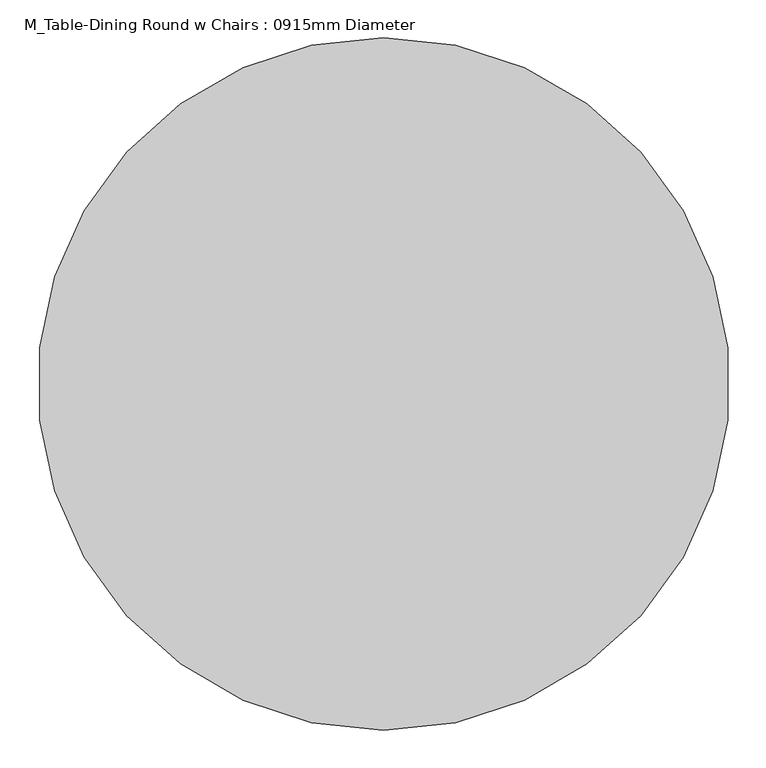
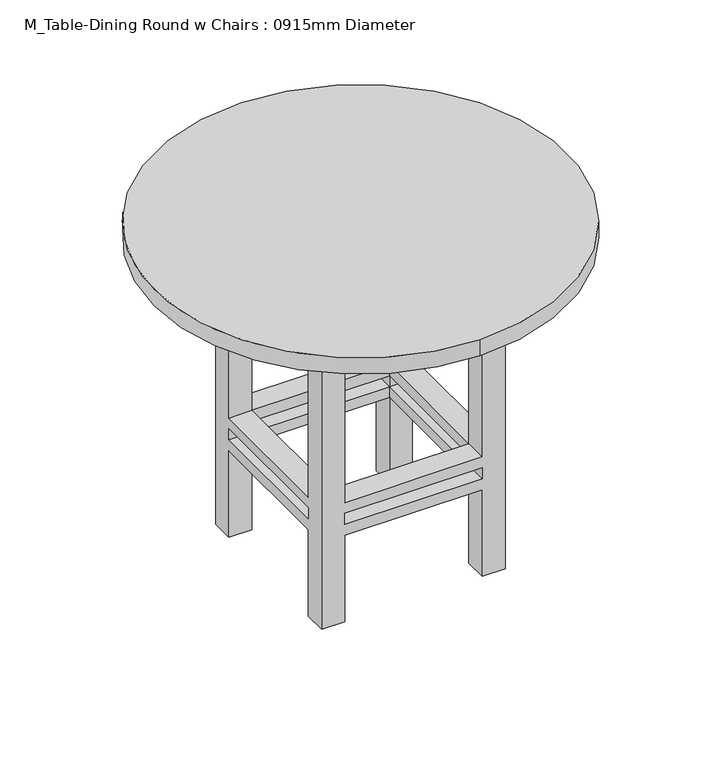
"""IFC4 building model written with IfcOpenShell, lengths in millimetres: furniture geometry, M_Table-Dining Round w Chairs : 0915mm Diameter."""

from ifc_helpers import new_model, si_unit, point, frame, frame_2d, origin, place, context, project, spatial, polyline, circle_curve, trimmed, segment, composite_curve, outline, extrude, faceted_brep, source, transform, mapped, element, save


def m_table_dining_round_w_chairs_0915mm_diameter_5defa876(model_context):
    return source(origin(), model_context, "Body", "SolidModel", [
        faceted_brep([(-48.8680328, 18.4713115, 647.7), (-99.6680328, 18.4713115, 647.7), (-99.6680328, -32.3286885, 647.7), (-48.8680328, -32.3286885, 647.7), (256.2319672, 18.4713115, 647.7), (256.2319672, -32.3286885, 647.7), (307.0319672, -32.3286885, 647.7), (307.0319672, 18.4713115, 647.7), (256.2319672, -388.2286885, 647.7), (307.0319672, -388.2286885, 647.7), (307.0319672, -337.4286885, 647.7), (256.2319672, -337.4286885, 647.7), (-48.8680328, -388.2286885, 647.7), (-48.8680328, -337.4286885, 647.7), (-99.6680328, -337.4286885, 647.7), (-99.6680328, -388.2286885, 647.7), (-48.8680328, 18.4713115, 0.0), (-48.8680328, -32.3286885, 0.0), (-99.6680328, -32.3286885, 0.0), (-99.6680328, 18.4713115, 0.0), (256.2319672, 18.4713115, 0.0), (307.0319672, 18.4713115, 0.0), (307.0319672, -32.3286885, 0.0), (256.2319672, -32.3286885, 0.0), (256.2319672, -388.2286885, 0.0), (256.2319672, -337.4286885, 0.0), (307.0319672, -337.4286885, 0.0), (307.0319672, -388.2286885, 0.0), (-48.8680328, -388.2286885, 0.0), (-99.6680328, -388.2286885, 0.0), (-99.6680328, -337.4286885, 0.0), (-48.8680328, -337.4286885, 0.0), (-48.8680328, 18.4713115, 279.4), (256.2319672, 18.4713115, 279.4), (256.2319672, 18.4713115, 203.2), (-48.8680328, 18.4713115, 203.2), (256.2319672, 18.4713115, 228.6), (256.2319672, 18.4713115, 254.0), (-48.8680328, 18.4713115, 254.0), (-48.8680328, 18.4713115, 228.6), (-99.6680328, -32.3286885, 203.2), (-99.6680328, -337.4286885, 203.2), (-99.6680328, -337.4286885, 279.4), (-99.6680328, -32.3286885, 279.4), (-99.6680328, -32.3286885, 228.6), (-99.6680328, -32.3286885, 254.0), (-99.6680328, -337.4286885, 254.0), (-99.6680328, -337.4286885, 228.6), (-48.8680328, -32.3286885, 279.4), (-48.8680328, -32.3286885, 203.2), (-48.8680328, -32.3286885, 228.6), (-48.8680328, -32.3286885, 254.0), (256.2319672, -32.3286885, 279.4), (256.2319672, -32.3286885, 203.2), (256.2319672, -32.3286885, 228.6), (256.2319672, -32.3286885, 254.0), (307.0319672, -32.3286885, 279.4), (307.0319672, -32.3286885, 203.2), (307.0319672, -32.3286885, 228.6), (307.0319672, -32.3286885, 254.0), (307.0319672, -337.4286885, 279.4), (307.0319672, -337.4286885, 203.2), (307.0319672, -337.4286885, 228.6), (307.0319672, -337.4286885, 254.0), (256.2319672, -388.2286885, 279.4), (-48.8680328, -388.2286885, 279.4), (-48.8680328, -388.2286885, 203.2), (256.2319672, -388.2286885, 203.2), (-48.8680328, -388.2286885, 228.6), (-48.8680328, -388.2286885, 254.0), (256.2319672, -388.2286885, 254.0), (256.2319672, -388.2286885, 228.6), (256.2319672, -337.4286885, 279.4), (256.2319672, -337.4286885, 203.2), (256.2319672, -337.4286885, 228.6), (256.2319672, -337.4286885, 254.0), (-48.8680328, -337.4286885, 279.4), (-48.8680328, -337.4286885, 203.2), (-48.8680328, -337.4286885, 228.6), (-48.8680328, -337.4286885, 254.0)], [[[0, 1, 2, 3]], [[4, 5, 6, 7]], [[8, 9, 10, 11]], [[12, 13, 14, 15]], [[16, 17, 18, 19]], [[20, 21, 22, 23]], [[24, 25, 26, 27]], [[28, 29, 30, 31]], [[1, 0, 32, 33, 4, 7, 21, 20, 34, 35, 16, 19], [36, 37, 38, 39]], [[2, 1, 19, 18, 40, 41, 30, 29, 15, 14, 42, 43], [44, 45, 46, 47]], [[3, 2, 43, 48]], [[18, 17, 49, 40]], [[44, 50, 51, 45]], [[0, 3, 48, 32]], [[17, 16, 35, 49]], [[50, 39, 38, 51]], [[5, 4, 33, 52]], [[20, 23, 53, 34]], [[36, 54, 55, 37]], [[6, 5, 52, 56]], [[23, 22, 57, 53]], [[54, 58, 59, 55]], [[21, 7, 6, 56, 60, 10, 9, 27, 26, 61, 57, 22], [62, 63, 59, 58]], [[27, 9, 8, 64, 65, 12, 15, 29, 28, 66, 67, 24], [68, 69, 70, 71]], [[11, 10, 60, 72]], [[26, 25, 73, 61]], [[62, 74, 75, 63]], [[8, 11, 72, 64]], [[25, 24, 67, 73]], [[74, 71, 70, 75]], [[13, 12, 65, 76]], [[28, 31, 77, 66]], [[68, 78, 79, 69]], [[14, 13, 76, 42]], [[31, 30, 41, 77]], [[78, 47, 46, 79]], [[54, 74, 62, 58]], [[74, 78, 68, 71]], [[78, 50, 44, 47]], [[50, 54, 36, 39]], [[53, 49, 35, 34]], [[49, 77, 41, 40]], [[77, 73, 67, 66]], [[73, 53, 57, 61]], [[74, 54, 53, 73]], [[78, 74, 73, 77]], [[50, 78, 77, 49]], [[54, 50, 49, 53]], [[52, 72, 60, 56]], [[72, 76, 65, 64]], [[76, 48, 43, 42]], [[48, 52, 33, 32]], [[55, 51, 38, 37]], [[51, 79, 46, 45]], [[79, 75, 70, 69]], [[75, 55, 59, 63]], [[72, 52, 55, 75]], [[76, 72, 75, 79]], [[48, 76, 79, 51]], [[52, 48, 51, 55]]]),
        extrude(outline(polyline([(332.4319672, 43.8713115), (332.4319672, -413.6286885), (-125.0680328, -413.6286885), (-125.0680328, 43.8713115), (332.4319672, 43.8713115)]), holes=[polyline([(307.0319672, 18.4713115), (-99.6680328, 18.4713115), (-99.6680328, -388.2286885), (307.0319672, -388.2286885), (307.0319672, 18.4713115)])]), frame((0.0, 0.0, 647.7), z_axis=(0.0, 0.0, 1.0), x_axis=(1.0, 0.0, 0.0)), (0.0, 0.0, 1.0), 76.2),
        extrude(outline(composite_curve([segment(trimmed(circle_curve(frame_2d((103.6819672, -184.8786885)), 457.5), [point((103.6819672, -642.3786885))], [point((103.6819672, 272.6213115))], False, "CARTESIAN"), True, "CONTINUOUS"), segment(trimmed(circle_curve(frame_2d((103.6819672, -184.8786885)), 457.5), [point((103.6819672, 272.6213115))], [point((103.6819672, -642.3786885))], False, "CARTESIAN"), True, "CONTINUOUS")], self_intersect=False)), frame((0.0, 0.0, 723.9), z_axis=(0.0, 0.0, 1.0), x_axis=(1.0, 0.0, 0.0)), (0.0, 0.0, 1.0), 38.1),
    ])


if __name__ == "__main__":
    model = new_model("IFC4")
    model_context = context("Model", 3, world=origin())
    ifc_project = project(units=[si_unit("LENGTHUNIT", "METRE", prefix="MILLI")], contexts=[model_context])
    site = spatial("IfcSite", under=ifc_project)
    building = spatial("IfcBuilding", under=site)
    placement = place(None, origin())
    m_table_dining_round_w_chairs_0915mm_diameter_shape = m_table_dining_round_w_chairs_0915mm_diameter_5defa876(model_context)
    element("IfcFurniture", 1, ObjectType="M_Table-Dining Round w Chairs : 0915mm Diameter", at=placement, inside=building, context=model_context, shape_type="MappedRepresentation", body=[
        mapped(m_table_dining_round_w_chairs_0915mm_diameter_shape, transform((0.0, 0.0, 0.0), x_axis=(1.0, 0.0, 0.0), y_axis=(0.0, 1.0, 0.0), z_axis=(0.0, 0.0, 1.0))),
    ])
    save(model, "model.ifc")

# Revit data of these elements
# Type "M_Table-Dining Round w Chairs : 0915mm Diameter"
#   Radius = 0.4575 m
#   Diameter = 0.915 m
#   Height = 0.762 m
#   Chairs = 4
#   Base Material = Pine
#   Top Material = Laminate, Linen, Matte
# Element 1 (IfcFurniture, "M_Table-Dining Round w Chairs : 0915mm Diameter")
#   Materials on its faces: "Pine", "Laminate, Linen, Matte"
# Materials
#   "Pine": class "Wood", colour RGB 223 192 134, transparency 0, Description = "Pinus Echinata", Cost = 0
#   "Laminate, Linen, Matte": class "Plastic", colour RGB 249 239 230, transparency 0, Description = "Plastic Laminate - Linen, Matte", Cost = 0
